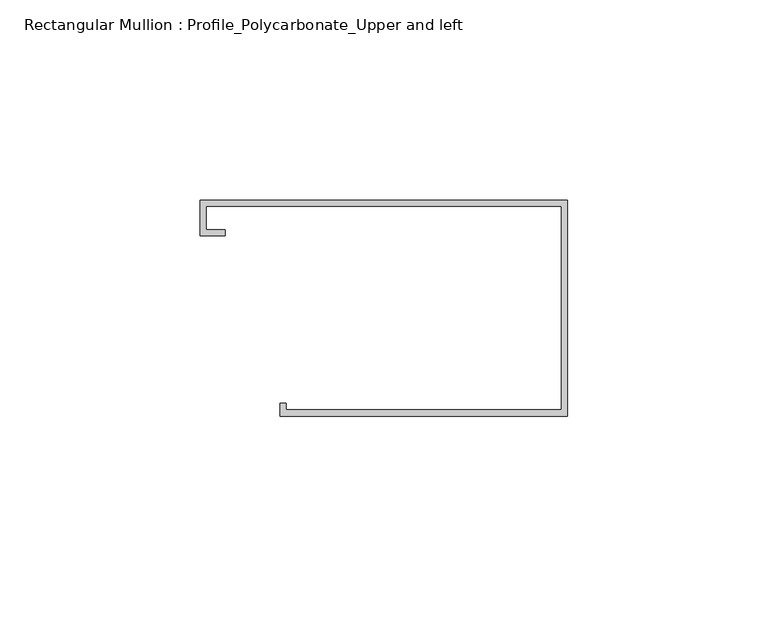
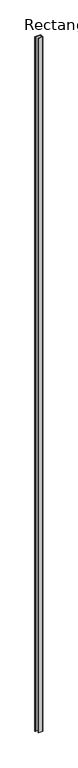
"""IFC4 building model written with IfcOpenShell, lengths in millimetres: member geometry, Rectangular Mullion : Profile_Polycarbonate_Upper and left."""

from ifc_helpers import new_model, si_unit, frame, origin, place, context, project, spatial, polyline, outline, extrude, source, transform, mapped, element, save


def rectangular_mullion_profile_polycarbonate_upper_and_left_203d5e48(model_context):
    return source(origin(), model_context, "Body", "SweptSolid", [
        extrude(outline(polyline([(0.0, 28.984575), (0.0, -25.015825), (-71.9836, -25.015825), (-71.9836, -21.840825), (-70.3961, -21.840825), (-70.3961, -23.428325), (-1.5875, -23.428325), (-1.5875, 27.397075), (-90.4113, 27.397075), (-90.4113, 21.580475), (-85.6488, 21.580475), (-85.6488, 19.992975), (-91.9988, 19.992975), (-91.9988, 28.984575), (0.0, 28.984575)])), frame((0.0, 0.0, -11382.5274), z_axis=(0.0, 0.0, 1.0), x_axis=(1.0, 0.0, 0.0)), (0.0, 0.0, 1.0), 11382.5274),
    ])


if __name__ == "__main__":
    model = new_model("IFC4")
    model_context = context("Model", 3, world=origin())
    ifc_project = project(units=[si_unit("LENGTHUNIT", "METRE", prefix="MILLI")], contexts=[model_context])
    site = spatial("IfcSite", under=ifc_project)
    building = spatial("IfcBuilding", under=site)
    placement = place(None, origin())
    rectangular_mullion_profile_polycarbonate_upper_and_left_shape = rectangular_mullion_profile_polycarbonate_upper_and_left_203d5e48(model_context)
    element("IfcMember", 1, ObjectType="Rectangular Mullion : Profile_Polycarbonate_Upper and left", at=placement, inside=building, context=model_context, shape_type="MappedRepresentation", body=[
        mapped(rectangular_mullion_profile_polycarbonate_upper_and_left_shape, transform((0.0, 0.0, 0.0), x_axis=(1.0, 0.0, 0.0), y_axis=(0.0, 1.0, 0.0), z_axis=(0.0, 0.0, 1.0))),
    ])
    save(model, "model.ifc")

# Revit data of these elements
# Type "Rectangular Mullion : Profile_Polycarbonate_Upper and left"
#   built-in parameter 1007322 = 0.177167 (stored number, unit not read)
#   built-in parameter 1007321 = 0.00520833 (stored number, unit not read)
#   built-in parameter 1007320 = 0 (stored number, unit not read)
